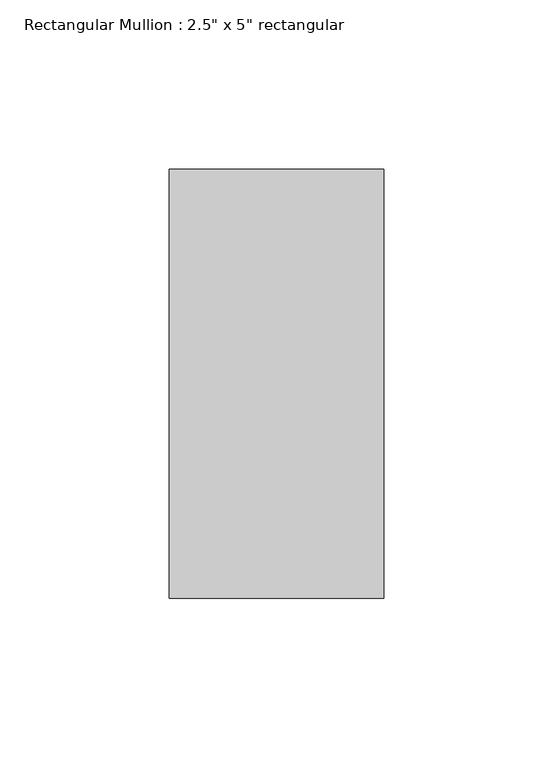
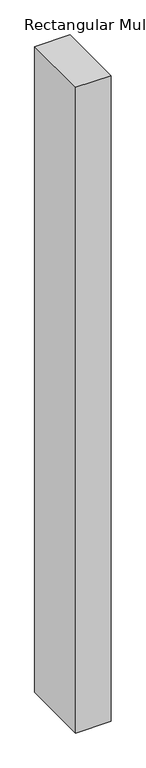
"""IFC4 building model written with IfcOpenShell, lengths in millimetres: member geometry."""

from ifc_helpers import new_model, si_unit, frame, origin, place, context, project, spatial, polyline, outline, extrude, source, transform, mapped, element, save


def member_28f0a790(model_context):
    return source(origin(), model_context, "Body", "SweptSolid", [
        extrude(outline(polyline([(0.0, 63.5), (0.0, -63.5), (-63.5, -63.5), (-63.5, 63.5), (0.0, 63.5)])), frame((0.0, 0.0, -1220.5651287), z_axis=(0.0, 0.0, 1.0), x_axis=(1.0, 0.0, 0.0)), (0.0, 0.0, 1.0), 1220.5651287),
    ])


if __name__ == "__main__":
    model = new_model("IFC4")
    model_context = context("Model", 3, world=origin())
    ifc_project = project(units=[si_unit("LENGTHUNIT", "METRE", prefix="MILLI")], contexts=[model_context])
    site = spatial("IfcSite", under=ifc_project)
    building = spatial("IfcBuilding", under=site)
    placement = place(None, origin())
    member_shape = member_28f0a790(model_context)
    element("IfcMember", 1, ObjectType="Rectangular Mullion : 2.5\" x 5\" rectangular", at=placement, inside=building, context=model_context, shape_type="MappedRepresentation", body=[
        mapped(member_shape, transform((0.0, 0.0, 0.0), x_axis=(1.0, 0.0, 0.0), y_axis=(0.0, 1.0, 0.0), z_axis=(0.0, 0.0, 1.0))),
    ])
    save(model, "model.ifc")

# Revit data of these elements
# Type "Rectangular Mullion : 2.5\" x 5\" rectangular"
#   built-in parameter 1007304 = 0.416667 (stored number, unit not read)
#   built-in parameter 1007301 = 0.104167 (stored number, unit not read)
#   built-in parameter 1007300 = 0.104167 (stored number, unit not read)
# Element 1 (IfcMember, "Rectangular Mullion : 2.5\" x 5\" rectangular")
#   Materials on its faces: "Metal - Aluminum"
# Materials
#   "Metal - Aluminum": class "Metal", colour RGB 140 140 140, transparency 0
